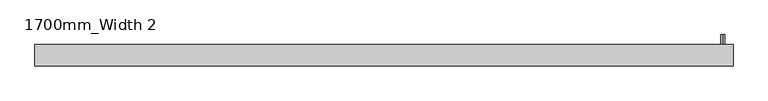
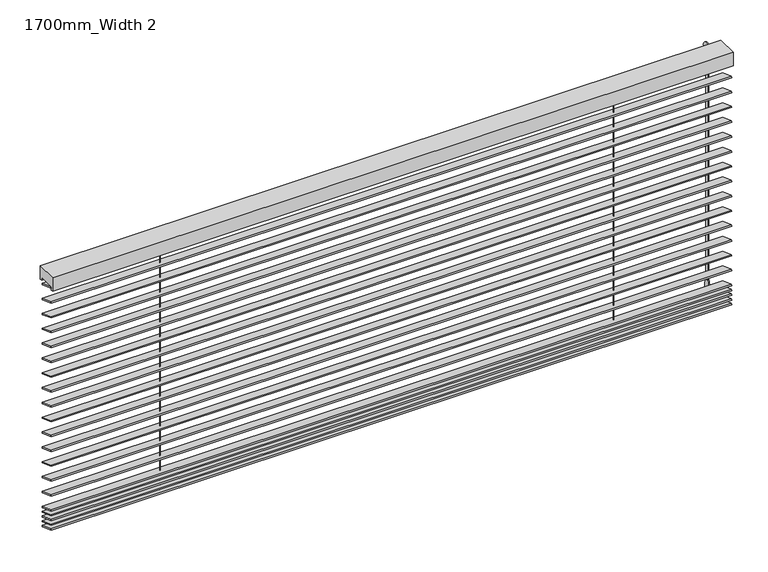
"""IFC4 building model written with IfcOpenShell, lengths in millimetres: proxy geometry, Specialty_Equipment_Venetian_Blind_Half_Down : 1700mm_Width 2."""

import ifcopenshell
import ifcopenshell.guid

model = None  # the IFC model being written
_history = None  # IfcOwnerHistory: only IFC2X3 demands one
_inside = {}  # id of a spatial element -> (the spatial element, [elements in it])
_under = {}  # id of a project, library or spatial element -> (it, [spatial elements below it])
_declared = {}  # id of a project -> (the project, [libraries it declares])
_typed = {}  # id of a type object -> (the type object, [elements of that type])
_made_of = {}  # id of a material, layer set ... -> (it, [elements and type objects made of it])


def new_model(schema):
    """Start an empty IFC model of exactly this schema.

    Asked for "IFC4X3", IfcOpenShell would pick the latest addendum, in which some entities
    have other attributes; the version numbers below select the first issue.
    IFC2X3 requires an IfcOwnerHistory on every rooted entity: one is made here for all.
    """
    global model, _history
    if schema == "IFC4X3":
        model = ifcopenshell.file(schema_version=(4, 3, 0, 0))
    else:
        model = ifcopenshell.file(schema=schema)
    _inside.clear()
    _under.clear()
    _declared.clear()
    _typed.clear()
    _made_of.clear()
    _history = None
    if model.schema == "IFC2X3":
        org = make("IfcOrganization", Name="unknown")
        user = make(
            "IfcPersonAndOrganization",
            ThePerson=make("IfcPerson", FamilyName="unknown"),
            TheOrganization=org,
        )
        app = make(
            "IfcApplication",
            ApplicationDeveloper=org,
            Version="unknown",
            ApplicationFullName="unknown",
            ApplicationIdentifier="unknown",
        )
        _history = make(
            "IfcOwnerHistory",
            OwningUser=user,
            OwningApplication=app,
            ChangeAction="ADDED",
            CreationDate=0,
        )
    return model


def make(cls, **values):
    """One entity of the class cls with the attributes given. An attribute that is None is left unset."""
    return model.create_entity(
        cls, **{name: value for name, value in values.items() if value is not None}
    )


def rooted(cls, **values):
    """An entity with a GlobalId (a new one), such as an element, a storey or a relation."""
    return make(cls, GlobalId=ifcopenshell.guid.new(), OwnerHistory=_history, **values)


def si_unit(unit_type, name, prefix=None):
    """IfcSIUnit, for example si_unit("LENGTHUNIT", "METRE", prefix="MILLI")."""
    return make("IfcSIUnit", UnitType=unit_type, Prefix=prefix, Name=name)


def assignment(units):
    """IfcUnitAssignment: the units of a project."""
    return None if units is None else make("IfcUnitAssignment", Units=units)


def point(xyz):
    """IfcCartesianPoint."""
    return None if xyz is None else make("IfcCartesianPoint", Coordinates=xyz)


def direction(xyz):
    """IfcDirection."""
    return None if xyz is None else make("IfcDirection", DirectionRatios=xyz)


def frame(location, z_axis=None, x_axis=None):
    """IfcAxis2Placement3D, a coordinate frame: its origin and axes. An axis left out is left unset."""
    return make(
        "IfcAxis2Placement3D",
        Location=point(location),
        Axis=direction(z_axis),
        RefDirection=direction(x_axis),
    )


def frame_2d(location, x_axis=None):
    """IfcAxis2Placement2D, a coordinate frame in the plane: its origin and x axis."""
    return make(
        "IfcAxis2Placement2D", Location=point(location), RefDirection=direction(x_axis)
    )


def origin():
    """The frame at (0, 0, 0) with its axes left unset."""
    return frame((0.0, 0.0, 0.0))


def place(relative_to, where):
    """IfcLocalPlacement: puts the frame where relative to a parent placement (None: the world)."""
    return make(
        "IfcLocalPlacement", PlacementRelTo=relative_to, RelativePlacement=where
    )


def context(
    kind, dimensions, precision=None, world=None, true_north=None, identifier=None
):
    """IfcGeometricRepresentationContext, for example the 3D "Model" context."""
    return make(
        "IfcGeometricRepresentationContext",
        ContextIdentifier=identifier,
        ContextType=kind,
        CoordinateSpaceDimension=dimensions,
        Precision=precision,
        WorldCoordinateSystem=world,
        TrueNorth=true_north,
    )


def project(units=None, contexts=None):
    """IfcProject with its units and contexts."""
    return rooted(
        "IfcProject",
        Name="project",
        RepresentationContexts=contexts,
        UnitsInContext=assignment(units),
    )


def spatial(cls, under=None, at=None, **own):
    """A site, building, storey or space (cls), placed at a placement, below another one or the project."""
    s = rooted(cls, ObjectPlacement=at, **own)
    if under is not None:
        _under.setdefault(under.id(), (under, []))[1].append(s)
    return s


def polyline(points):
    """IfcPolyline through the points."""
    return make("IfcPolyline", Points=[point(p) for p in points])


def circle_curve(where, radius):
    """IfcCircle in the frame where."""
    return make("IfcCircle", Position=where, Radius=radius)


def ellipse_curve(where, semi_axis1, semi_axis2):
    """IfcEllipse in the frame where."""
    return make(
        "IfcEllipse", Position=where, SemiAxis1=semi_axis1, SemiAxis2=semi_axis2
    )


def trimmed(basis, trim1, trim2, sense, master):
    """IfcTrimmedCurve: the piece of a basis curve between two trims."""
    return make(
        "IfcTrimmedCurve",
        BasisCurve=basis,
        Trim1=trim1,
        Trim2=trim2,
        SenseAgreement=sense,
        MasterRepresentation=master,
    )


def segment(curve, same_sense, transition):
    """IfcCompositeCurveSegment."""
    return make(
        "IfcCompositeCurveSegment",
        Transition=transition,
        SameSense=same_sense,
        ParentCurve=curve,
    )


def composite_curve(segments, self_intersect=None):
    """IfcCompositeCurve: segments joined end to end."""
    return make("IfcCompositeCurve", Segments=segments, SelfIntersect=self_intersect)


def outline(outer, holes=None, kind="AREA"):
    """IfcArbitraryClosedProfileDef: a profile drawn as a closed curve; with holes, ...WithVoids."""
    if holes is None:
        return make("IfcArbitraryClosedProfileDef", ProfileType=kind, OuterCurve=outer)
    return make(
        "IfcArbitraryProfileDefWithVoids",
        ProfileType=kind,
        OuterCurve=outer,
        InnerCurves=holes,
    )


def extrude(swept, where, along, depth):
    """IfcExtrudedAreaSolid: the profile swept, set in the frame where, extruded along a direction by depth."""
    return make(
        "IfcExtrudedAreaSolid",
        SweptArea=swept,
        Position=where,
        ExtrudedDirection=direction(along),
        Depth=depth,
    )


def shape(context_of_items, identifier, shape_type, items):
    """IfcShapeRepresentation: the items that make up one representation, for example the "Body"."""
    return make(
        "IfcShapeRepresentation",
        ContextOfItems=context_of_items,
        RepresentationIdentifier=identifier,
        RepresentationType=shape_type,
        Items=items,
    )


def source(mapping_origin, context_of_items, identifier, shape_type, items):
    """IfcRepresentationMap: a shape defined once, which mapped items show again and again."""
    return make(
        "IfcRepresentationMap",
        MappingOrigin=mapping_origin,
        MappedRepresentation=shape(context_of_items, identifier, shape_type, items),
    )


def transform(
    local_origin,
    x_axis=None,
    y_axis=None,
    z_axis=None,
    scale=None,
    scale2=None,
    scale3=None,
    uniform=True,
):
    """IfcCartesianTransformationOperator3D, or its non-uniform kind. x_axis, y_axis, z_axis: its Axis1, 2, 3."""
    if uniform:
        return make(
            "IfcCartesianTransformationOperator3D",
            Axis1=direction(x_axis),
            Axis2=direction(y_axis),
            LocalOrigin=point(local_origin),
            Scale=scale,
            Axis3=direction(z_axis),
        )
    return make(
        "IfcCartesianTransformationOperator3DnonUniform",
        Axis1=direction(x_axis),
        Axis2=direction(y_axis),
        LocalOrigin=point(local_origin),
        Scale=scale,
        Axis3=direction(z_axis),
        Scale2=scale2,
        Scale3=scale3,
    )


def mapped(mapping_source, mapping_target):
    """IfcMappedItem: shows the shape of a source again, moved by a transform."""
    return make(
        "IfcMappedItem", MappingSource=mapping_source, MappingTarget=mapping_target
    )


def made_of(thing, what):
    """Note that an element or type object is made of a material, layer set ...; save() writes the relation."""
    if what is not None:
        _made_of.setdefault(what.id(), (what, []))[1].append(thing)
    return thing


def element(
    cls,
    number,
    at=None,
    inside=None,
    cuts=None,
    type_object=None,
    material=None,
    context=None,
    identifier="Body",
    shape_type=None,
    held_by="IfcProductDefinitionShape",
    body=None,
    shapes=None,
    **own,
):
    """One element of the class cls, such as IfcWall. Its Tag is "e" and its number.

    at: its placement. inside: the storey or other place that contains it. cuts: it is an
    opening in that element (IfcRelVoidsElement). A single representation is given by context,
    identifier, shape_type and body (its items); several are given by shapes. held_by: the class
    of the entity that holds the representations. save() writes the other relations.
    """
    e = rooted(cls, Tag="e%d" % number, ObjectPlacement=at, **own)
    if body is not None:
        shapes = [shape(context, identifier, shape_type, body)]
    if shapes is not None:
        e.Representation = make(held_by, Representations=shapes)
    if inside is not None:
        _inside.setdefault(inside.id(), (inside, []))[1].append(e)
    if cuts is not None:
        rooted(
            "IfcRelVoidsElement", RelatingBuildingElement=cuts, RelatedOpeningElement=e
        )
    if type_object is not None:
        _typed.setdefault(type_object.id(), (type_object, []))[1].append(e)
    return made_of(e, material)


def aggregate(whole, parts):
    """IfcRelAggregates: a whole, such as a stair, and the parts it consists of."""
    return rooted("IfcRelAggregates", RelatingObject=whole, RelatedObjects=parts)


def save(model, path):
    """Write the relations noted so far, then the file.

    IfcRelAggregates (storeys below a building ...), IfcRelContainedInSpatialStructure (elements
    in a storey), IfcRelDefinesByType, IfcRelAssociatesMaterial and IfcRelDeclares: one each for
    every whole, place, type object, material and project.
    """
    for whole, parts in _under.values():
        aggregate(whole, parts)
    for where, things in _inside.values():
        rooted(
            "IfcRelContainedInSpatialStructure",
            RelatedElements=things,
            RelatingStructure=where,
        )
    for kind, things in _typed.values():
        rooted("IfcRelDefinesByType", RelatedObjects=things, RelatingType=kind)
    for what, things in _made_of.values():
        rooted("IfcRelAssociatesMaterial", RelatedObjects=things, RelatingMaterial=what)
    for by, libraries in _declared.values():
        rooted("IfcRelDeclares", RelatingContext=by, RelatedDefinitions=libraries)
    model.write(path)


def plane_surface(at):
    """IfcPlane: the flat surface through the origin of the frame at, square to its z axis."""
    return make("IfcPlane", Position=at)


def cylinder_surface(at, radius):
    """IfcCylindricalSurface: all points at the distance radius from the z axis of the frame at."""
    return make("IfcCylindricalSurface", Position=at, Radius=radius)


def revolved_surface(curve, axis_point, axis_direction):
    """IfcSurfaceOfRevolution: the curve turned about the line through axis_point along axis_direction."""
    return make(
        "IfcSurfaceOfRevolution",
        SweptCurve=make("IfcArbitraryOpenProfileDef", ProfileType="CURVE", Curve=curve),
        AxisPosition=make("IfcAxis1Placement", Location=point(axis_point), Axis=direction(axis_direction)),
    )


def advanced_brep(points, edges, surfaces, faces):
    """IfcAdvancedBrep: a solid bounded by faces that lie on surfaces and meet in shared edges.

    An edge is (start, end): straight between two places in points (the first is 0);
    or (start, end, curve); or (start, end, curve, False) where it runs against its curve.
    A face is (place in surfaces, loops), or (place, loops, False) where it looks against
    its surface's normal. A loop lists edges by number (the first is 1), with a minus sign
    where the edge is run from its end to its start. The first loop is the outer one.
    """
    corners = [point(p) for p in points]
    vertices = [make("IfcVertexPoint", VertexGeometry=c) for c in corners]
    made = []
    for start, end, *more in edges:
        made.append(
            make(
                "IfcEdgeCurve",
                EdgeStart=vertices[start],
                EdgeEnd=vertices[end],
                EdgeGeometry=more[0] if more else make("IfcPolyline", Points=[corners[start], corners[end]]),
                SameSense=more[1] if len(more) > 1 else True,
            )
        )
    hull = []
    for where, loops, *sense in faces:
        bounds = []
        for j, loop in enumerate(loops):
            ring = [make("IfcOrientedEdge", EdgeElement=made[abs(k) - 1], Orientation=k > 0) for k in loop]
            bounds.append(
                make(
                    "IfcFaceOuterBound" if j == 0 else "IfcFaceBound",
                    Bound=make("IfcEdgeLoop", EdgeList=ring),
                    Orientation=True,
                )
            )
        hull.append(make("IfcAdvancedFace", Bounds=bounds, FaceSurface=surfaces[where], SameSense=sense[0] if sense else True))
    return make("IfcAdvancedBrep", Outer=make("IfcClosedShell", CfsFaces=hull))


def proxy_1700mm_width_2_f283f02f(model_context):
    return source(origin(), model_context, "Body", "SolidModel", [
        extrude(outline(polyline([(0.0, 40.0), (1680.0, 40.0), (1680.0, 0.0), (0.0, 0.0), (0.0, 40.0)])), frame((-689.5079376, -65.0532351, 1447.7279746), z_axis=(0.0, 0.3420201433256684, 0.9396926207859085), x_axis=(1.0, 0.0, 0.0)), (0.0, 0.0, 1.0), 3.0625345),
        extrude(outline(polyline([(0.0, 40.0), (1680.0, 40.0), (1680.0, 0.0), (0.0, 0.0), (0.0, 40.0)])), frame((-689.5079376, -65.0532351, 1459.9116214), z_axis=(0.0, 0.3420201433256684, 0.9396926207859085), x_axis=(1.0, 0.0, 0.0)), (0.0, 0.0, 1.0), 3.0625345),
        extrude(outline(polyline([(0.0, 40.0), (1680.0, 40.0), (1680.0, 0.0), (0.0, 0.0), (0.0, 40.0)])), frame((-689.5079376, -65.0532351, 1472.7202682), z_axis=(0.0, 0.3420201433256684, 0.9396926207859085), x_axis=(1.0, 0.0, 0.0)), (0.0, 0.0, 1.0), 3.0625345),
        extrude(outline(polyline([(0.0, 40.0), (1680.0, 40.0), (1680.0, 0.0), (0.0, 0.0), (0.0, 40.0)])), frame((-689.5079376, -65.0532351, 1484.903915), z_axis=(0.0, 0.3420201433256684, 0.9396926207859085), x_axis=(1.0, 0.0, 0.0)), (0.0, 0.0, 1.0), 3.0625345),
        extrude(outline(polyline([(0.0, 40.0), (1680.0, 40.0), (1680.0, 0.0), (0.0, 0.0), (0.0, 40.0)])), frame((-689.5079376, -65.0532351, 2040.2125618), z_axis=(0.0, 0.3420201433256684, 0.9396926207859085), x_axis=(1.0, 0.0, 0.0)), (0.0, 0.0, 1.0), 3.0625345),
        extrude(outline(polyline([(0.0, 40.0), (1680.0, 40.0), (1680.0, 0.0), (0.0, 0.0), (0.0, 40.0)])), frame((-689.5079376, -65.0532351, 2001.4625618), z_axis=(0.0, 0.3420201433256684, 0.9396926207859085), x_axis=(1.0, 0.0, 0.0)), (0.0, 0.0, 1.0), 3.0625345),
        extrude(outline(polyline([(0.0, 40.0), (1680.0, 40.0), (1680.0, 0.0), (0.0, 0.0), (0.0, 40.0)])), frame((-689.5079376, -65.0532351, 1962.7125618), z_axis=(0.0, 0.3420201433256684, 0.9396926207859085), x_axis=(1.0, 0.0, 0.0)), (0.0, 0.0, 1.0), 3.0625345),
        extrude(outline(polyline([(0.0, 40.0), (1680.0, 40.0), (1680.0, 0.0), (0.0, 0.0), (0.0, 40.0)])), frame((-689.5079376, -65.0532351, 1923.9625618), z_axis=(0.0, 0.3420201433256684, 0.9396926207859085), x_axis=(1.0, 0.0, 0.0)), (0.0, 0.0, 1.0), 3.0625345),
        extrude(outline(polyline([(0.0, 40.0), (1680.0, 40.0), (1680.0, 0.0), (0.0, 0.0), (0.0, 40.0)])), frame((-689.5079376, -65.0532351, 1885.2125618), z_axis=(0.0, 0.3420201433256684, 0.9396926207859085), x_axis=(1.0, 0.0, 0.0)), (0.0, 0.0, 1.0), 3.0625345),
        extrude(outline(polyline([(0.0, 40.0), (1680.0, 40.0), (1680.0, 0.0), (0.0, 0.0), (0.0, 40.0)])), frame((-689.5079376, -65.0532351, 1846.4625618), z_axis=(0.0, 0.3420201433256684, 0.9396926207859085), x_axis=(1.0, 0.0, 0.0)), (0.0, 0.0, 1.0), 3.0625345),
        extrude(outline(polyline([(0.0, 40.0), (1680.0, 40.0), (1680.0, 0.0), (0.0, 0.0), (0.0, 40.0)])), frame((-689.5079376, -65.0532351, 1807.7125618), z_axis=(0.0, 0.3420201433256684, 0.9396926207859085), x_axis=(1.0, 0.0, 0.0)), (0.0, 0.0, 1.0), 3.0625345),
        extrude(outline(polyline([(0.0, 40.0), (1680.0, 40.0), (1680.0, 0.0), (0.0, 0.0), (0.0, 40.0)])), frame((-689.5079376, -65.0532351, 1768.9625618), z_axis=(0.0, 0.3420201433256684, 0.9396926207859085), x_axis=(1.0, 0.0, 0.0)), (0.0, 0.0, 1.0), 3.0625345),
        extrude(outline(polyline([(0.0, 40.0), (1680.0, 40.0), (1680.0, 0.0), (0.0, 0.0), (0.0, 40.0)])), frame((-689.5079376, -65.0532351, 1730.2125618), z_axis=(0.0, 0.3420201433256684, 0.9396926207859085), x_axis=(1.0, 0.0, 0.0)), (0.0, 0.0, 1.0), 3.0625345),
        extrude(outline(polyline([(0.0, 40.0), (1680.0, 40.0), (1680.0, 0.0), (0.0, 0.0), (0.0, 40.0)])), frame((-689.5079376, -65.0532351, 1691.4625618), z_axis=(0.0, 0.3420201433256684, 0.9396926207859085), x_axis=(1.0, 0.0, 0.0)), (0.0, 0.0, 1.0), 3.0625345),
        extrude(outline(polyline([(0.0, 40.0), (1680.0, 40.0), (1680.0, 0.0), (0.0, 0.0), (0.0, 40.0)])), frame((-689.5079376, -65.0532351, 1652.7125618), z_axis=(0.0, 0.3420201433256684, 0.9396926207859085), x_axis=(1.0, 0.0, 0.0)), (0.0, 0.0, 1.0), 3.0625345),
        extrude(outline(polyline([(0.0, 40.0), (1680.0, 40.0), (1680.0, 0.0), (0.0, 0.0), (0.0, 40.0)])), frame((-689.5079376, -65.0532351, 1613.9625618), z_axis=(0.0, 0.3420201433256684, 0.9396926207859085), x_axis=(1.0, 0.0, 0.0)), (0.0, 0.0, 1.0), 3.0625345),
        extrude(outline(polyline([(0.0, 40.0), (1680.0, 40.0), (1680.0, 0.0), (0.0, 0.0), (0.0, 40.0)])), frame((-689.5079376, -65.0532351, 1575.2125618), z_axis=(0.0, 0.3420201433256684, 0.9396926207859085), x_axis=(1.0, 0.0, 0.0)), (0.0, 0.0, 1.0), 3.0625345),
        extrude(outline(polyline([(0.0, 40.0), (1680.0, 40.0), (1680.0, 0.0), (0.0, 0.0), (0.0, 40.0)])), frame((-689.5079376, -65.0532351, 1536.4625618), z_axis=(0.0, 0.3420201433256684, 0.9396926207859085), x_axis=(1.0, 0.0, 0.0)), (0.0, 0.0, 1.0), 3.0625345),
        extrude(outline(polyline([(0.0, 40.0), (1680.0, 40.0), (1680.0, 0.0), (0.0, 0.0), (0.0, 40.0)])), frame((-689.5079376, -65.0532351, 1497.7125618), z_axis=(0.0, 0.3420201433256684, 0.9396926207859085), x_axis=(1.0, 0.0, 0.0)), (0.0, 0.0, 1.0), 3.0625345),
        extrude(outline(polyline([(0.0, 40.0), (1680.0, 40.0), (1680.0, 0.0), (0.0, 0.0), (0.0, 40.0)])), frame((-689.5079376, -65.0532351, 2078.9625618), z_axis=(0.0, 0.3420201433256684, 0.9396926207859085), x_axis=(1.0, 0.0, 0.0)), (0.0, 0.0, 1.0), 3.0625345),
        extrude(outline(composite_curve([segment(trimmed(circle_curve(frame_2d((-409.5079376, -45.2119342)), 0.5), [point((-410.0079376, -45.2119342))], [point((-409.0079376, -45.2119342))], False, "CARTESIAN"), True, "CONTINUOUS"), segment(trimmed(circle_curve(frame_2d((-409.5079376, -45.2119342)), 0.5), [point((-409.0079376, -45.2119342))], [point((-410.0079376, -45.2119342))], False, "CARTESIAN"), True, "CONTINUOUS")], self_intersect=False)), frame((0.0, 0.0, 1434.9736305), z_axis=(0.0, 0.0, 1.0), x_axis=(1.0, 0.0, 0.0)), (0.0, 0.0, 1.0), 648.2712578),
        extrude(outline(composite_curve([segment(trimmed(circle_curve(frame_2d((710.4920624, -45.2119342)), 0.5), [point((709.9920624, -45.2119342))], [point((710.9920624, -45.2119342))], False, "CARTESIAN"), True, "CONTINUOUS"), segment(trimmed(circle_curve(frame_2d((710.4920624, -45.2119342)), 0.5), [point((710.9920624, -45.2119342))], [point((709.9920624, -45.2119342))], False, "CARTESIAN"), True, "CONTINUOUS")], self_intersect=False)), frame((0.0, 0.0, 1434.9736305), z_axis=(0.0, 0.0, 1.0), x_axis=(1.0, 0.0, 0.0)), (0.0, 0.0, 1.0), 648.2712578),
        advanced_brep(
        [(965.4920624, -4.7248495, 2091.3243671), (965.4920624, -3.7248495, 2091.3243671), (965.4920624, -2.7248495, 2091.3243671), (965.4920624, -4.7248495, 2076.3243671), (965.4920624, -2.7248495, 2076.3243671), (965.4920624, -6.7248495, 2076.3243671), (965.4920624, -0.7248495, 2076.3243671), (965.4920624, -6.7248495, 1486.909931), (965.4920624, -0.7248495, 1486.909931), (965.4920624, -7.2513368, 1460.0), (965.4920624, -0.1983622, 1460.0), (965.4920624, -3.7248495, 1460.0)],
        [
            (0, 1),
            (1, 2),
            (2, 0, circle_curve(frame((965.4920624, -3.7248495, 2091.3243671), z_axis=(0.0, 0.0, 1.0), x_axis=(0.0, 1.0, 0.0)), 1.0)),
            (0, 2, circle_curve(frame((965.4920624, -3.7248495, 2091.3243671), z_axis=(0.0, 0.0, 1.0), x_axis=(0.0, 1.0, 0.0)), 1.0)),
            (3, 0),
            (2, 4),
            (4, 3, circle_curve(frame((965.4920624, -3.7248495, 2076.3243671), z_axis=(0.0, 0.0, 1.0), x_axis=(0.0, 1.0, 0.0)), 1.0)),
            (3, 4, circle_curve(frame((965.4920624, -3.7248495, 2076.3243671), z_axis=(0.0, 0.0, 1.0), x_axis=(0.0, 1.0, 0.0)), 1.0)),
            (5, 3),
            (4, 6),
            (6, 5, circle_curve(frame((965.4920624, -3.7248495, 2076.3243671), z_axis=(0.0, 0.0, 1.0), x_axis=(0.0, 1.0, 0.0)), 3.0)),
            (5, 6, circle_curve(frame((965.4920624, -3.7248495, 2076.3243671), z_axis=(0.0, 0.0, 1.0), x_axis=(0.0, 1.0, 0.0)), 3.0)),
            (7, 5),
            (6, 8),
            (8, 7, circle_curve(frame((965.4920624, -3.7248495, 1486.909931), z_axis=(0.0, 0.0, 1.0), x_axis=(0.0, 1.0, 0.0)), 3.0)),
            (7, 8, circle_curve(frame((965.4920624, -3.7248495, 1486.909931), z_axis=(0.0, 0.0, 1.0), x_axis=(0.0, 1.0, 0.0)), 3.0)),
            (9, 7, circle_curve(frame((965.4920624, 41.8223072, 1472.5), z_axis=(-1.0, 0.0, 0.0), x_axis=(0.0, 1.0, 0.0)), 50.6406214)),
            (8, 10, circle_curve(frame((965.4920624, -49.2720063, 1472.5), z_axis=(-1.0, 0.0, 0.0), x_axis=(0.0, -1.0, 0.0)), 50.6406214)),
            (10, 9, circle_curve(frame((965.4920624, -3.7248495, 1460.0), z_axis=(0.0, 0.0, 1.0), x_axis=(0.0, 1.0, 0.0)), 3.5264873)),
            (9, 10, circle_curve(frame((965.4920624, -3.7248495, 1460.0), z_axis=(0.0, 0.0, 1.0), x_axis=(0.0, 1.0, 0.0)), 3.5264873)),
            (11, 9),
            (10, 11),
        ],
        [
            plane_surface(frame((965.4920624, -3.7248495, 2091.3243671), z_axis=(0.0, 0.0, 1.0), x_axis=(0.0, 1.0, 0.0))),
            cylinder_surface(frame((965.4920624, -3.7248495, 1191.3243671), z_axis=(0.0, 0.0, -1.0), x_axis=(0.0, 1.0, 0.0)), 1.0),
            plane_surface(frame((965.4920624, -3.7248495, 2076.3243671), z_axis=(0.0, 0.0, 1.0), x_axis=(0.0, 1.0, 0.0))),
            cylinder_surface(frame((965.4920624, -3.7248495, 1191.3243671), z_axis=(0.0, 0.0, -1.0), x_axis=(0.0, 1.0, 0.0)), 3.0),
            revolved_surface(trimmed(ellipse_curve(frame((965.4920624, -49.2720063, 1472.5), z_axis=(-1.0, 0.0, 0.0), x_axis=(0.0, -1.0, 0.0)), 50.6406214, 50.6406214), [point((965.4920624, -0.7248495, 1486.909931))], [point((965.4920624, -0.1983622, 1460.0))], True, "CARTESIAN"), (965.4920624, -3.7248495, 1191.3243671), (0.0, 0.0, -1.0)),
            plane_surface(frame((965.4920624, -3.7248495, 1460.0), z_axis=(0.0, 0.0, -1.0), x_axis=(0.0, 1.0, 0.0))),
        ],
        [
            (0, [[1, 2, 3]]),
            (0, [[-2, -1, 4]]),
            (1, [[5, -3, 6, 7]]),
            (1, [[-6, -4, -5, 8]]),
            (2, [[9, -7, 10, 11]]),
            (2, [[-10, -8, -9, 12]]),
            (3, [[13, -11, 14, 15]]),
            (3, [[-14, -12, -13, 16]]),
            (4, [[17, -15, 18, 19]]),
            (4, [[-18, -16, -17, 20]]),
            (5, [[21, -19, 22]]),
            (5, [[-22, -20, -21]]),
        ],
    ),
        extrude(outline(composite_curve([segment(trimmed(circle_curve(frame_2d((2095.9171213, 965.4920624)), 5.0), [point((2100.9171213, 965.4920624))], [point((2090.9171213, 965.4920624))], False, "CARTESIAN"), True, "CONTINUOUS"), segment(trimmed(circle_curve(frame_2d((2095.9171213, 965.4920624)), 5.0), [point((2090.9171213, 965.4920624))], [point((2100.9171213, 965.4920624))], False, "CARTESIAN"), True, "CONTINUOUS")], self_intersect=False)), frame((0.0, -19.329714, 0.0), z_axis=(0.0, 1.0, 0.0), x_axis=(0.0, 0.0, 1.0)), (0.0, 0.0, 1.0), 23.7809602),
        extrude(outline(polyline([(-19.329714, 2110.0), (-19.329714, 2075.0), (-24.329714, 2075.0), (-24.329714, 2083.2448883), (-66.0941545, 2083.2448883), (-66.0941545, 2075.0), (-71.0941545, 2075.0), (-71.0941545, 2110.0), (-19.329714, 2110.0)])), frame((-689.5079376, 0.0, 0.0), z_axis=(1.0, 0.0, 0.0), x_axis=(0.0, 1.0, 0.0)), (0.0, 0.0, 1.0), 1680.0),
    ])


if __name__ == "__main__":
    model = new_model("IFC4")
    model_context = context("Model", 3, world=origin())
    ifc_project = project(units=[si_unit("LENGTHUNIT", "METRE", prefix="MILLI")], contexts=[model_context])
    site = spatial("IfcSite", under=ifc_project)
    building = spatial("IfcBuilding", under=site)
    placement = place(None, origin())
    proxy_1700mm_width_2_shape = proxy_1700mm_width_2_f283f02f(model_context)
    element("IfcBuildingElementProxy", 1, Name="Specialty_Equipment_Venetian_Blind_Half_Down : 1700mm_Width 2", ObjectType="Specialty_Equipment_Venetian_Blind_Half_Down : 1700mm_Width 2", at=placement, inside=building, context=model_context, shape_type="MappedRepresentation", body=[
        mapped(proxy_1700mm_width_2_shape, transform((0.0, 0.0, 0.0), x_axis=(1.0, 0.0, 0.0), y_axis=(0.0, 1.0, 0.0), z_axis=(0.0, 0.0, 1.0))),
    ])
    save(model, "model.ifc")

# Revit data of these elements
# Type "Specialty_Equipment_Venetian_Blind_Half_Down : 1700mm_Width 2"
#   Keynote = "N10/240"
#   Opening Width = 1700 mm
#   End Offset = 10 mm
#   Blind Length = 1680 mm
#   Blind Fixing Height = 2110 mm
#   Blind Depth = 980 mm
#   Blind Angle = 20.00°
#   Blade Depth = 40 mm
#   No of Blades = 25
#   Material Blind = Wood - Birch
#   Default Elevation = 0
# Element 1 (IfcBuildingElementProxy, "Specialty_Equipment_Venetian_Blind_Half_Down : 1700mm_Width 2")
#   Materials on its faces: "Wood - Birch"
# Materials
#   "Wood - Birch": class "Wood", colour RGB 224 178 126, transparency 0
